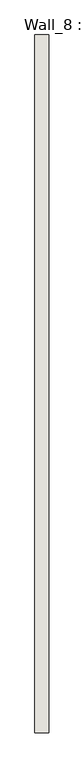
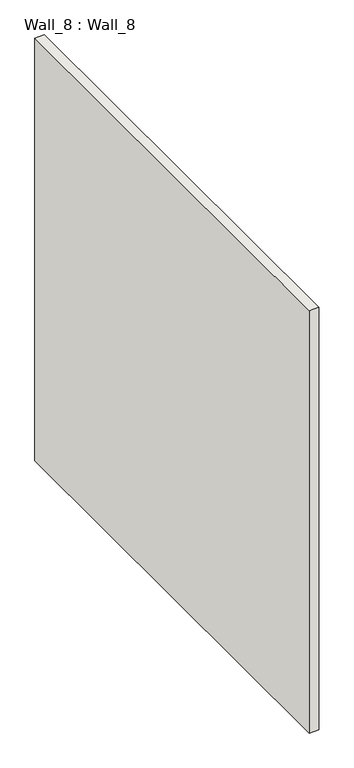
"""IFC4 building model written with IfcOpenShell, lengths in millimetres: wall geometry, Wall_8 : Wall_8."""

from ifc_helpers import new_model, si_unit, origin, origin_with_axes, place, context, project, spatial, polyline, outline, extrude, source, transform, mapped, element, save


def wall_8_wall_8_015fc5ca(model_context):
    return source(origin(), model_context, "Body", "SweptSolid", [
        extrude(outline(polyline([(6290.0, 16990.0), (6290.0, 11990.0), (6190.0, 11990.0), (6190.0, 16990.0), (6290.0, 16990.0)])), origin_with_axes(), (0.0, 0.0, 1.0), 4700.0),
    ])


if __name__ == "__main__":
    model = new_model("IFC4")
    model_context = context("Model", 3, world=origin())
    ifc_project = project(units=[si_unit("LENGTHUNIT", "METRE", prefix="MILLI")], contexts=[model_context])
    site = spatial("IfcSite", under=ifc_project)
    building = spatial("IfcBuilding", under=site)
    placement = place(None, origin())
    wall_8_wall_8_shape = wall_8_wall_8_015fc5ca(model_context)
    element("IfcWall", 1, ObjectType="Wall_8 : Wall_8", at=placement, inside=building, context=model_context, shape_type="MappedRepresentation", body=[
        mapped(wall_8_wall_8_shape, transform((0.0, 0.0, 0.0), x_axis=(1.0, 0.0, 0.0), y_axis=(0.0, 1.0, 0.0), z_axis=(0.0, 0.0, 1.0))),
    ])
    save(model, "model.ifc")

# Revit data of these elements
# Type "Wall_8 : Wall_8"
#   NameOverride = "Wall_8"
# Element 1 (IfcWall, "Wall_8 : Wall_8")
#   Materials on its faces: "IfcSurfaceStyle #33"
# Materials
#   "IfcSurfaceStyle #33": class "Unassigned", colour RGB 214 214 214, transparency 0
